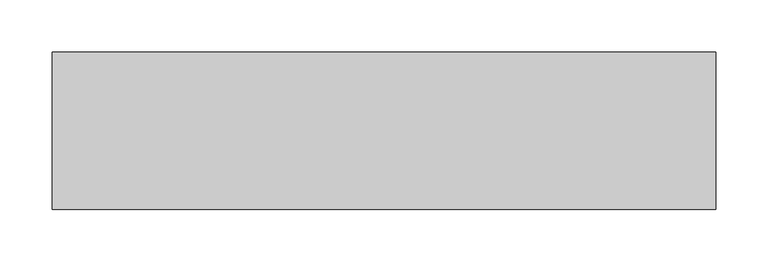
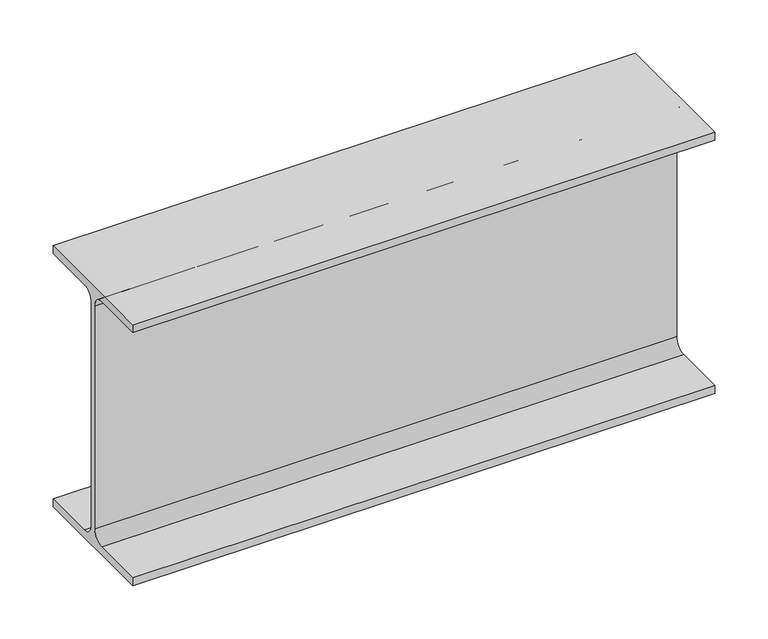
"""IFC4 building model written with IfcOpenShell, lengths in millimetres: beam geometry, 0912_Steel Framing_H-KSD3502 : H_SB_ASB_H-300x150x6.5x9."""

import ifcopenshell
import ifcopenshell.guid

model = None  # the IFC model being written
_history = None  # IfcOwnerHistory: only IFC2X3 demands one
_inside = {}  # id of a spatial element -> (the spatial element, [elements in it])
_under = {}  # id of a project, library or spatial element -> (it, [spatial elements below it])
_declared = {}  # id of a project -> (the project, [libraries it declares])
_typed = {}  # id of a type object -> (the type object, [elements of that type])
_made_of = {}  # id of a material, layer set ... -> (it, [elements and type objects made of it])


def new_model(schema):
    """Start an empty IFC model of exactly this schema.

    Asked for "IFC4X3", IfcOpenShell would pick the latest addendum, in which some entities
    have other attributes; the version numbers below select the first issue.
    IFC2X3 requires an IfcOwnerHistory on every rooted entity: one is made here for all.
    """
    global model, _history
    if schema == "IFC4X3":
        model = ifcopenshell.file(schema_version=(4, 3, 0, 0))
    else:
        model = ifcopenshell.file(schema=schema)
    _inside.clear()
    _under.clear()
    _declared.clear()
    _typed.clear()
    _made_of.clear()
    _history = None
    if model.schema == "IFC2X3":
        org = make("IfcOrganization", Name="unknown")
        user = make(
            "IfcPersonAndOrganization",
            ThePerson=make("IfcPerson", FamilyName="unknown"),
            TheOrganization=org,
        )
        app = make(
            "IfcApplication",
            ApplicationDeveloper=org,
            Version="unknown",
            ApplicationFullName="unknown",
            ApplicationIdentifier="unknown",
        )
        _history = make(
            "IfcOwnerHistory",
            OwningUser=user,
            OwningApplication=app,
            ChangeAction="ADDED",
            CreationDate=0,
        )
    return model


def make(cls, **values):
    """One entity of the class cls with the attributes given. An attribute that is None is left unset."""
    return model.create_entity(
        cls, **{name: value for name, value in values.items() if value is not None}
    )


def rooted(cls, **values):
    """An entity with a GlobalId (a new one), such as an element, a storey or a relation."""
    return make(cls, GlobalId=ifcopenshell.guid.new(), OwnerHistory=_history, **values)


def si_unit(unit_type, name, prefix=None):
    """IfcSIUnit, for example si_unit("LENGTHUNIT", "METRE", prefix="MILLI")."""
    return make("IfcSIUnit", UnitType=unit_type, Prefix=prefix, Name=name)


def assignment(units):
    """IfcUnitAssignment: the units of a project."""
    return None if units is None else make("IfcUnitAssignment", Units=units)


def point(xyz):
    """IfcCartesianPoint."""
    return None if xyz is None else make("IfcCartesianPoint", Coordinates=xyz)


def direction(xyz):
    """IfcDirection."""
    return None if xyz is None else make("IfcDirection", DirectionRatios=xyz)


def frame(location, z_axis=None, x_axis=None):
    """IfcAxis2Placement3D, a coordinate frame: its origin and axes. An axis left out is left unset."""
    return make(
        "IfcAxis2Placement3D",
        Location=point(location),
        Axis=direction(z_axis),
        RefDirection=direction(x_axis),
    )


def frame_2d(location, x_axis=None):
    """IfcAxis2Placement2D, a coordinate frame in the plane: its origin and x axis."""
    return make(
        "IfcAxis2Placement2D", Location=point(location), RefDirection=direction(x_axis)
    )


def origin():
    """The frame at (0, 0, 0) with its axes left unset."""
    return frame((0.0, 0.0, 0.0))


def place(relative_to, where):
    """IfcLocalPlacement: puts the frame where relative to a parent placement (None: the world)."""
    return make(
        "IfcLocalPlacement", PlacementRelTo=relative_to, RelativePlacement=where
    )


def context(
    kind, dimensions, precision=None, world=None, true_north=None, identifier=None
):
    """IfcGeometricRepresentationContext, for example the 3D "Model" context."""
    return make(
        "IfcGeometricRepresentationContext",
        ContextIdentifier=identifier,
        ContextType=kind,
        CoordinateSpaceDimension=dimensions,
        Precision=precision,
        WorldCoordinateSystem=world,
        TrueNorth=true_north,
    )


def project(units=None, contexts=None):
    """IfcProject with its units and contexts."""
    return rooted(
        "IfcProject",
        Name="project",
        RepresentationContexts=contexts,
        UnitsInContext=assignment(units),
    )


def spatial(cls, under=None, at=None, **own):
    """A site, building, storey or space (cls), placed at a placement, below another one or the project."""
    s = rooted(cls, ObjectPlacement=at, **own)
    if under is not None:
        _under.setdefault(under.id(), (under, []))[1].append(s)
    return s


def polyline(points):
    """IfcPolyline through the points."""
    return make("IfcPolyline", Points=[point(p) for p in points])


def circle_curve(where, radius):
    """IfcCircle in the frame where."""
    return make("IfcCircle", Position=where, Radius=radius)


def trimmed(basis, trim1, trim2, sense, master):
    """IfcTrimmedCurve: the piece of a basis curve between two trims."""
    return make(
        "IfcTrimmedCurve",
        BasisCurve=basis,
        Trim1=trim1,
        Trim2=trim2,
        SenseAgreement=sense,
        MasterRepresentation=master,
    )


def segment(curve, same_sense, transition):
    """IfcCompositeCurveSegment."""
    return make(
        "IfcCompositeCurveSegment",
        Transition=transition,
        SameSense=same_sense,
        ParentCurve=curve,
    )


def composite_curve(segments, self_intersect=None):
    """IfcCompositeCurve: segments joined end to end."""
    return make("IfcCompositeCurve", Segments=segments, SelfIntersect=self_intersect)


def outline(outer, holes=None, kind="AREA"):
    """IfcArbitraryClosedProfileDef: a profile drawn as a closed curve; with holes, ...WithVoids."""
    if holes is None:
        return make("IfcArbitraryClosedProfileDef", ProfileType=kind, OuterCurve=outer)
    return make(
        "IfcArbitraryProfileDefWithVoids",
        ProfileType=kind,
        OuterCurve=outer,
        InnerCurves=holes,
    )


def extrude(swept, where, along, depth):
    """IfcExtrudedAreaSolid: the profile swept, set in the frame where, extruded along a direction by depth."""
    return make(
        "IfcExtrudedAreaSolid",
        SweptArea=swept,
        Position=where,
        ExtrudedDirection=direction(along),
        Depth=depth,
    )


def shape(context_of_items, identifier, shape_type, items):
    """IfcShapeRepresentation: the items that make up one representation, for example the "Body"."""
    return make(
        "IfcShapeRepresentation",
        ContextOfItems=context_of_items,
        RepresentationIdentifier=identifier,
        RepresentationType=shape_type,
        Items=items,
    )


def source(mapping_origin, context_of_items, identifier, shape_type, items):
    """IfcRepresentationMap: a shape defined once, which mapped items show again and again."""
    return make(
        "IfcRepresentationMap",
        MappingOrigin=mapping_origin,
        MappedRepresentation=shape(context_of_items, identifier, shape_type, items),
    )


def transform(
    local_origin,
    x_axis=None,
    y_axis=None,
    z_axis=None,
    scale=None,
    scale2=None,
    scale3=None,
    uniform=True,
):
    """IfcCartesianTransformationOperator3D, or its non-uniform kind. x_axis, y_axis, z_axis: its Axis1, 2, 3."""
    if uniform:
        return make(
            "IfcCartesianTransformationOperator3D",
            Axis1=direction(x_axis),
            Axis2=direction(y_axis),
            LocalOrigin=point(local_origin),
            Scale=scale,
            Axis3=direction(z_axis),
        )
    return make(
        "IfcCartesianTransformationOperator3DnonUniform",
        Axis1=direction(x_axis),
        Axis2=direction(y_axis),
        LocalOrigin=point(local_origin),
        Scale=scale,
        Axis3=direction(z_axis),
        Scale2=scale2,
        Scale3=scale3,
    )


def mapped(mapping_source, mapping_target):
    """IfcMappedItem: shows the shape of a source again, moved by a transform."""
    return make(
        "IfcMappedItem", MappingSource=mapping_source, MappingTarget=mapping_target
    )


def made_of(thing, what):
    """Note that an element or type object is made of a material, layer set ...; save() writes the relation."""
    if what is not None:
        _made_of.setdefault(what.id(), (what, []))[1].append(thing)
    return thing


def element(
    cls,
    number,
    at=None,
    inside=None,
    cuts=None,
    type_object=None,
    material=None,
    context=None,
    identifier="Body",
    shape_type=None,
    held_by="IfcProductDefinitionShape",
    body=None,
    shapes=None,
    **own,
):
    """One element of the class cls, such as IfcWall. Its Tag is "e" and its number.

    at: its placement. inside: the storey or other place that contains it. cuts: it is an
    opening in that element (IfcRelVoidsElement). A single representation is given by context,
    identifier, shape_type and body (its items); several are given by shapes. held_by: the class
    of the entity that holds the representations. save() writes the other relations.
    """
    e = rooted(cls, Tag="e%d" % number, ObjectPlacement=at, **own)
    if body is not None:
        shapes = [shape(context, identifier, shape_type, body)]
    if shapes is not None:
        e.Representation = make(held_by, Representations=shapes)
    if inside is not None:
        _inside.setdefault(inside.id(), (inside, []))[1].append(e)
    if cuts is not None:
        rooted(
            "IfcRelVoidsElement", RelatingBuildingElement=cuts, RelatedOpeningElement=e
        )
    if type_object is not None:
        _typed.setdefault(type_object.id(), (type_object, []))[1].append(e)
    return made_of(e, material)


def aggregate(whole, parts):
    """IfcRelAggregates: a whole, such as a stair, and the parts it consists of."""
    return rooted("IfcRelAggregates", RelatingObject=whole, RelatedObjects=parts)


def save(model, path):
    """Write the relations noted so far, then the file.

    IfcRelAggregates (storeys below a building ...), IfcRelContainedInSpatialStructure (elements
    in a storey), IfcRelDefinesByType, IfcRelAssociatesMaterial and IfcRelDeclares: one each for
    every whole, place, type object, material and project.
    """
    for whole, parts in _under.values():
        aggregate(whole, parts)
    for where, things in _inside.values():
        rooted(
            "IfcRelContainedInSpatialStructure",
            RelatedElements=things,
            RelatingStructure=where,
        )
    for kind, things in _typed.values():
        rooted("IfcRelDefinesByType", RelatedObjects=things, RelatingType=kind)
    for what, things in _made_of.values():
        rooted("IfcRelAssociatesMaterial", RelatedObjects=things, RelatingMaterial=what)
    for by, libraries in _declared.values():
        rooted("IfcRelDeclares", RelatingContext=by, RelatedDefinitions=libraries)
    model.write(path)


def beam_2895a1d0(model_context):
    return source(origin(), model_context, "Body", "SweptSolid", [
        extrude(outline(composite_curve([segment(polyline([(75.0, -141.0), (75.0, -150.0), (-75.0, -150.0), (-75.0, -141.0), (-16.25, -141.0)]), True, "CONTINUOUS"), segment(trimmed(circle_curve(frame_2d((-16.25, -128.0)), 13.0), [point((-16.25, -141.0))], [point((-3.25, -128.0))], True, "CARTESIAN"), True, "CONTINUOUS"), segment(polyline([(-3.25, -128.0), (-3.25, 128.0)]), True, "CONTINUOUS"), segment(trimmed(circle_curve(frame_2d((-16.25, 128.0)), 13.0), [point((-3.25, 128.0))], [point((-16.25, 141.0))], True, "CARTESIAN"), True, "CONTINUOUS"), segment(polyline([(-16.25, 141.0), (-75.0, 141.0), (-75.0, 150.0), (75.0, 150.0), (75.0, 141.0), (16.25, 141.0)]), True, "CONTINUOUS"), segment(trimmed(circle_curve(frame_2d((16.25, 128.0)), 13.0), [point((16.25, 141.0))], [point((3.25, 128.0))], True, "CARTESIAN"), True, "CONTINUOUS"), segment(polyline([(3.25, 128.0), (3.25, -128.0)]), True, "CONTINUOUS"), segment(trimmed(circle_curve(frame_2d((16.25, -128.0)), 13.0), [point((3.25, -128.0))], [point((16.25, -141.0))], True, "CARTESIAN"), True, "CONTINUOUS"), segment(polyline([(16.25, -141.0), (75.0, -141.0)]), True, "CONTINUOUS")], self_intersect=False)), frame((-282.3, 0.0, 0.0), z_axis=(1.0, 0.0, 0.0), x_axis=(0.0, 1.0, 0.0)), (0.0, 0.0, 1.0), 632.1),
    ])


if __name__ == "__main__":
    model = new_model("IFC4")
    model_context = context("Model", 3, world=origin())
    ifc_project = project(units=[si_unit("LENGTHUNIT", "METRE", prefix="MILLI")], contexts=[model_context])
    site = spatial("IfcSite", under=ifc_project)
    building = spatial("IfcBuilding", under=site)
    placement = place(None, origin())
    beam_shape = beam_2895a1d0(model_context)
    element("IfcBeam", 1, ObjectType="0912_Steel Framing_H-KSD3502 : H_SB_ASB_H-300x150x6.5x9", at=placement, inside=building, context=model_context, shape_type="MappedRepresentation", body=[
        mapped(beam_shape, transform((0.0, 0.0, 0.0), x_axis=(1.0, 0.0, 0.0), y_axis=(0.0, 1.0, 0.0), z_axis=(0.0, 0.0, 1.0))),
    ])
    save(model, "model.ifc")

# Revit data of these elements
# Type "0912_Steel Framing_H-KSD3502 : H_SB_ASB_H-300x150x6.5x9"
#   H_WM Code_1 = "S01AA002-00001 | Main Steel Structure Fabrication Work | Shelter/Building | Medium Steel - Standard (90KG/M>Weight≥30KG/M) | Material: (   )"
#   H_WM Code_2 = "S03AA028-00001 | Main Steel Structure Erection Work | Shelter/Building | Medium Steel (90KG/M>Weight≥30KG/M) | Material: (   )"
#   H_WM Code_3 = "S01AA010-00001 | Main Steel Structure Fabrication Work | Shelter/Building | Steel Painting/Coating | for Non-Fireproofed Steel Surface, Surface Preparation, Primer, Second & Final Coat | Material: (   )"
#   H_Q'ty Cal Type Tag = "SB-Q2"
#   Width = 15.0 cm
#   Web Thickness = 0.65 cm
#   Web Fillet = 1.3 cm
#   Warping Constant = 107000.0 cm⁶
#   W = 0
#   Torsional Moment of Inertia = 9.9539 cm⁴
#   Section Area = 46.78 cm²
#   Plastic Modulus weak axis = 105.0 cm³
#   Plastic Modulus strong axis = 542.0 cm³
#   Perimeter = 1.17 m²/m
#   Nominal Weight = 36.70 kgf/m
#   Moment of Inertia weak axis = 508.00 cm⁴
#   Moment of Inertia strong axis = 7210.00 cm⁴
#   Height = 30.0 cm
#   Flange Thickness = 0.9 cm
#   Elastic Modulus weak axis = 67.7 cm³
#   Elastic Modulus strong axis = 481.0 cm³
#   Centroid Vertical = 15.0 cm
#   Centroid Horizontal = 7.5 cm
#   Ix = 72100000
#   Length [instance default] = 1.5240 m
#   Zx = 542000
#   b = 0.1500 m
#   h = 0.3000 m
#   r = 0.0130 m
#   s = 0.0065 m
#   t = 0.0090 m
#   A = 0.004678 m²
#   Structural Material [instance default] = Steel, 45-345
#   Assembly Code = ""
# Element 1 (IfcBeam, "0912_Steel Framing_H-KSD3502 : H_SB_ASB_H-300x150x6.5x9")
#   Structural Material = none
# Materials
#   "Steel, 45-345": class "Metal", colour RGB 189 187 185, transparency 0, Description = "Steel 345 MPa", Cost = 0
